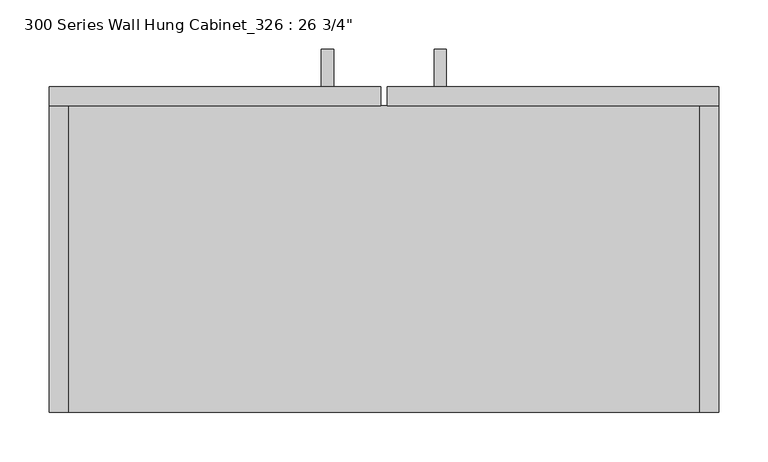
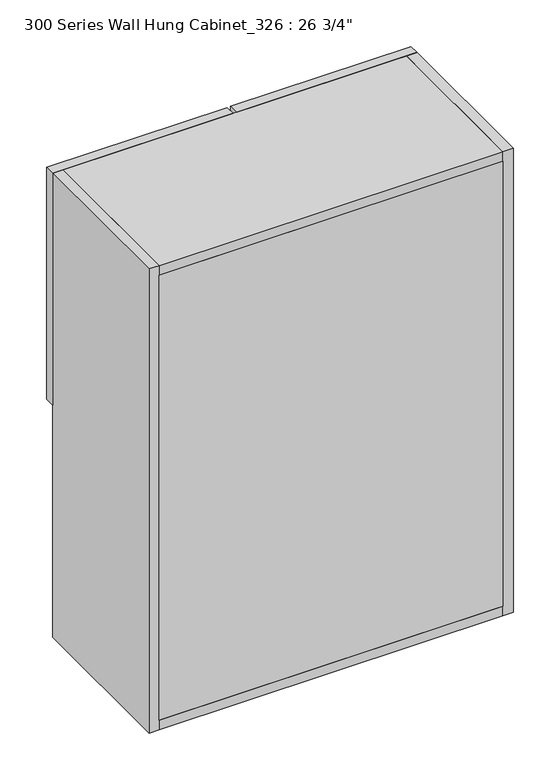
"""IFC4 building model written with IfcOpenShell, lengths in millimetres: furniture geometry."""

import ifcopenshell
import ifcopenshell.guid

model = None  # the IFC model being written
_history = None  # IfcOwnerHistory: only IFC2X3 demands one
_inside = {}  # id of a spatial element -> (the spatial element, [elements in it])
_under = {}  # id of a project, library or spatial element -> (it, [spatial elements below it])
_declared = {}  # id of a project -> (the project, [libraries it declares])
_typed = {}  # id of a type object -> (the type object, [elements of that type])
_made_of = {}  # id of a material, layer set ... -> (it, [elements and type objects made of it])


def new_model(schema):
    """Start an empty IFC model of exactly this schema.

    Asked for "IFC4X3", IfcOpenShell would pick the latest addendum, in which some entities
    have other attributes; the version numbers below select the first issue.
    IFC2X3 requires an IfcOwnerHistory on every rooted entity: one is made here for all.
    """
    global model, _history
    if schema == "IFC4X3":
        model = ifcopenshell.file(schema_version=(4, 3, 0, 0))
    else:
        model = ifcopenshell.file(schema=schema)
    _inside.clear()
    _under.clear()
    _declared.clear()
    _typed.clear()
    _made_of.clear()
    _history = None
    if model.schema == "IFC2X3":
        org = make("IfcOrganization", Name="unknown")
        user = make(
            "IfcPersonAndOrganization",
            ThePerson=make("IfcPerson", FamilyName="unknown"),
            TheOrganization=org,
        )
        app = make(
            "IfcApplication",
            ApplicationDeveloper=org,
            Version="unknown",
            ApplicationFullName="unknown",
            ApplicationIdentifier="unknown",
        )
        _history = make(
            "IfcOwnerHistory",
            OwningUser=user,
            OwningApplication=app,
            ChangeAction="ADDED",
            CreationDate=0,
        )
    return model


def make(cls, **values):
    """One entity of the class cls with the attributes given. An attribute that is None is left unset."""
    return model.create_entity(
        cls, **{name: value for name, value in values.items() if value is not None}
    )


def rooted(cls, **values):
    """An entity with a GlobalId (a new one), such as an element, a storey or a relation."""
    return make(cls, GlobalId=ifcopenshell.guid.new(), OwnerHistory=_history, **values)


def si_unit(unit_type, name, prefix=None):
    """IfcSIUnit, for example si_unit("LENGTHUNIT", "METRE", prefix="MILLI")."""
    return make("IfcSIUnit", UnitType=unit_type, Prefix=prefix, Name=name)


def assignment(units):
    """IfcUnitAssignment: the units of a project."""
    return None if units is None else make("IfcUnitAssignment", Units=units)


def point(xyz):
    """IfcCartesianPoint."""
    return None if xyz is None else make("IfcCartesianPoint", Coordinates=xyz)


def direction(xyz):
    """IfcDirection."""
    return None if xyz is None else make("IfcDirection", DirectionRatios=xyz)


def frame(location, z_axis=None, x_axis=None):
    """IfcAxis2Placement3D, a coordinate frame: its origin and axes. An axis left out is left unset."""
    return make(
        "IfcAxis2Placement3D",
        Location=point(location),
        Axis=direction(z_axis),
        RefDirection=direction(x_axis),
    )


def origin():
    """The frame at (0, 0, 0) with its axes left unset."""
    return frame((0.0, 0.0, 0.0))


def place(relative_to, where):
    """IfcLocalPlacement: puts the frame where relative to a parent placement (None: the world)."""
    return make(
        "IfcLocalPlacement", PlacementRelTo=relative_to, RelativePlacement=where
    )


def context(
    kind, dimensions, precision=None, world=None, true_north=None, identifier=None
):
    """IfcGeometricRepresentationContext, for example the 3D "Model" context."""
    return make(
        "IfcGeometricRepresentationContext",
        ContextIdentifier=identifier,
        ContextType=kind,
        CoordinateSpaceDimension=dimensions,
        Precision=precision,
        WorldCoordinateSystem=world,
        TrueNorth=true_north,
    )


def project(units=None, contexts=None):
    """IfcProject with its units and contexts."""
    return rooted(
        "IfcProject",
        Name="project",
        RepresentationContexts=contexts,
        UnitsInContext=assignment(units),
    )


def spatial(cls, under=None, at=None, **own):
    """A site, building, storey or space (cls), placed at a placement, below another one or the project."""
    s = rooted(cls, ObjectPlacement=at, **own)
    if under is not None:
        _under.setdefault(under.id(), (under, []))[1].append(s)
    return s


def polyline(points):
    """IfcPolyline through the points."""
    return make("IfcPolyline", Points=[point(p) for p in points])


def outline(outer, holes=None, kind="AREA"):
    """IfcArbitraryClosedProfileDef: a profile drawn as a closed curve; with holes, ...WithVoids."""
    if holes is None:
        return make("IfcArbitraryClosedProfileDef", ProfileType=kind, OuterCurve=outer)
    return make(
        "IfcArbitraryProfileDefWithVoids",
        ProfileType=kind,
        OuterCurve=outer,
        InnerCurves=holes,
    )


def extrude(swept, where, along, depth):
    """IfcExtrudedAreaSolid: the profile swept, set in the frame where, extruded along a direction by depth."""
    return make(
        "IfcExtrudedAreaSolid",
        SweptArea=swept,
        Position=where,
        ExtrudedDirection=direction(along),
        Depth=depth,
    )


def shape(context_of_items, identifier, shape_type, items):
    """IfcShapeRepresentation: the items that make up one representation, for example the "Body"."""
    return make(
        "IfcShapeRepresentation",
        ContextOfItems=context_of_items,
        RepresentationIdentifier=identifier,
        RepresentationType=shape_type,
        Items=items,
    )


def source(mapping_origin, context_of_items, identifier, shape_type, items):
    """IfcRepresentationMap: a shape defined once, which mapped items show again and again."""
    return make(
        "IfcRepresentationMap",
        MappingOrigin=mapping_origin,
        MappedRepresentation=shape(context_of_items, identifier, shape_type, items),
    )


def transform(
    local_origin,
    x_axis=None,
    y_axis=None,
    z_axis=None,
    scale=None,
    scale2=None,
    scale3=None,
    uniform=True,
):
    """IfcCartesianTransformationOperator3D, or its non-uniform kind. x_axis, y_axis, z_axis: its Axis1, 2, 3."""
    if uniform:
        return make(
            "IfcCartesianTransformationOperator3D",
            Axis1=direction(x_axis),
            Axis2=direction(y_axis),
            LocalOrigin=point(local_origin),
            Scale=scale,
            Axis3=direction(z_axis),
        )
    return make(
        "IfcCartesianTransformationOperator3DnonUniform",
        Axis1=direction(x_axis),
        Axis2=direction(y_axis),
        LocalOrigin=point(local_origin),
        Scale=scale,
        Axis3=direction(z_axis),
        Scale2=scale2,
        Scale3=scale3,
    )


def mapped(mapping_source, mapping_target):
    """IfcMappedItem: shows the shape of a source again, moved by a transform."""
    return make(
        "IfcMappedItem", MappingSource=mapping_source, MappingTarget=mapping_target
    )


def made_of(thing, what):
    """Note that an element or type object is made of a material, layer set ...; save() writes the relation."""
    if what is not None:
        _made_of.setdefault(what.id(), (what, []))[1].append(thing)
    return thing


def element(
    cls,
    number,
    at=None,
    inside=None,
    cuts=None,
    type_object=None,
    material=None,
    context=None,
    identifier="Body",
    shape_type=None,
    held_by="IfcProductDefinitionShape",
    body=None,
    shapes=None,
    **own,
):
    """One element of the class cls, such as IfcWall. Its Tag is "e" and its number.

    at: its placement. inside: the storey or other place that contains it. cuts: it is an
    opening in that element (IfcRelVoidsElement). A single representation is given by context,
    identifier, shape_type and body (its items); several are given by shapes. held_by: the class
    of the entity that holds the representations. save() writes the other relations.
    """
    e = rooted(cls, Tag="e%d" % number, ObjectPlacement=at, **own)
    if body is not None:
        shapes = [shape(context, identifier, shape_type, body)]
    if shapes is not None:
        e.Representation = make(held_by, Representations=shapes)
    if inside is not None:
        _inside.setdefault(inside.id(), (inside, []))[1].append(e)
    if cuts is not None:
        rooted(
            "IfcRelVoidsElement", RelatingBuildingElement=cuts, RelatedOpeningElement=e
        )
    if type_object is not None:
        _typed.setdefault(type_object.id(), (type_object, []))[1].append(e)
    return made_of(e, material)


def aggregate(whole, parts):
    """IfcRelAggregates: a whole, such as a stair, and the parts it consists of."""
    return rooted("IfcRelAggregates", RelatingObject=whole, RelatedObjects=parts)


def save(model, path):
    """Write the relations noted so far, then the file.

    IfcRelAggregates (storeys below a building ...), IfcRelContainedInSpatialStructure (elements
    in a storey), IfcRelDefinesByType, IfcRelAssociatesMaterial and IfcRelDeclares: one each for
    every whole, place, type object, material and project.
    """
    for whole, parts in _under.values():
        aggregate(whole, parts)
    for where, things in _inside.values():
        rooted(
            "IfcRelContainedInSpatialStructure",
            RelatedElements=things,
            RelatingStructure=where,
        )
    for kind, things in _typed.values():
        rooted("IfcRelDefinesByType", RelatedObjects=things, RelatingType=kind)
    for what, things in _made_of.values():
        rooted("IfcRelAssociatesMaterial", RelatedObjects=things, RelatingMaterial=what)
    for by, libraries in _declared.values():
        rooted("IfcRelDeclares", RelatingContext=by, RelatedDefinitions=libraries)
    model.write(path)


def furniture_b195cdbb(model_context):
    return source(origin(), model_context, "Body", "SweptSolid", [
        extrude(outline(polyline([(406.4, 1809.7425373), (406.4, 1822.4121874), (444.4810937, 1822.4121874), (444.4810937, 1727.2), (406.4, 1727.2), (406.4, 1739.8696501), (431.8114436, 1739.8696501), (431.8114436, 1809.7425373), (406.4, 1809.7425373)])), frame((50.8, 0.0, 0.0), z_axis=(1.0, 0.0, 0.0), x_axis=(0.0, 1.0, 0.0)), (0.0, 0.0, 1.0), 12.4065288),
        extrude(outline(polyline([(406.4, 1809.7425373), (406.4, 1822.4121874), (444.4810937, 1822.4121874), (444.4810937, 1727.2), (406.4, 1727.2), (406.4, 1739.8696501), (431.8114436, 1739.8696501), (431.8114436, 1809.7425373), (406.4, 1809.7425373)])), frame((-63.5, 0.0, 0.0), z_axis=(1.0, 0.0, 0.0), x_axis=(0.0, 1.0, 0.0)), (0.0, 0.0, 1.0), 12.4065288),
        extrude(outline(polyline([(320.675, 387.35), (320.675, 95.25), (-320.675, 95.25), (-320.675, 387.35), (320.675, 387.35)])), frame((0.0, 0.0, 1676.4), z_axis=(0.0, 0.0, 1.0), x_axis=(1.0, 0.0, 0.0)), (0.0, 0.0, 1.0), 19.05),
        extrude(outline(polyline([(320.675, 76.2), (-320.675, 76.2), (-320.675, 95.25), (320.675, 95.25), (320.675, 76.2)])), frame((0.0, 0.0, 1238.25), z_axis=(0.0, 0.0, 1.0), x_axis=(1.0, 0.0, 0.0)), (0.0, 0.0, 1.0), 876.3),
        extrude(outline(polyline([(-3.175, 387.35), (-339.725, 387.35), (-339.725, 406.4), (-3.175, 406.4), (-3.175, 387.35)])), frame((0.0, 0.0, 1676.4), z_axis=(0.0, 0.0, 1.0), x_axis=(1.0, 0.0, 0.0)), (0.0, 0.0, 1.0), 457.2),
        extrude(outline(polyline([(339.725, 387.35), (3.175, 387.35), (3.175, 406.4), (339.725, 406.4), (339.725, 387.35)])), frame((0.0, 0.0, 1676.4), z_axis=(0.0, 0.0, 1.0), x_axis=(1.0, 0.0, 0.0)), (0.0, 0.0, 1.0), 457.2),
        extrude(outline(polyline([(-339.725, 76.2), (-339.725, 387.35), (-320.675, 387.35), (-320.675, 76.2), (-339.725, 76.2)])), frame((0.0, 0.0, 1219.2), z_axis=(0.0, 0.0, 1.0), x_axis=(1.0, 0.0, 0.0)), (0.0, 0.0, 1.0), 914.4),
        extrude(outline(polyline([(320.675, 76.2), (320.675, 387.35), (339.725, 387.35), (339.725, 76.2), (320.675, 76.2)])), frame((0.0, 0.0, 1219.2), z_axis=(0.0, 0.0, 1.0), x_axis=(1.0, 0.0, 0.0)), (0.0, 0.0, 1.0), 914.4),
        extrude(outline(polyline([(320.675, 387.35), (320.675, 76.2), (-320.675, 76.2), (-320.675, 387.35), (320.675, 387.35)])), frame((0.0, 0.0, 2114.55), z_axis=(0.0, 0.0, 1.0), x_axis=(1.0, 0.0, 0.0)), (0.0, 0.0, 1.0), 19.05),
        extrude(outline(polyline([(320.675, 387.35), (320.675, 76.2), (-320.675, 76.2), (-320.675, 387.35), (320.675, 387.35)])), frame((0.0, 0.0, 1219.2), z_axis=(0.0, 0.0, 1.0), x_axis=(1.0, 0.0, 0.0)), (0.0, 0.0, 1.0), 19.05),
    ])


if __name__ == "__main__":
    model = new_model("IFC4")
    model_context = context("Model", 3, world=origin())
    ifc_project = project(units=[si_unit("LENGTHUNIT", "METRE", prefix="MILLI")], contexts=[model_context])
    site = spatial("IfcSite", under=ifc_project)
    building = spatial("IfcBuilding", under=site)
    placement = place(None, origin())
    furniture_shape = furniture_b195cdbb(model_context)
    element("IfcFurniture", 1, ObjectType="300 Series Wall Hung Cabinet_326 : 26 3/4\"", at=placement, inside=building, context=model_context, shape_type="MappedRepresentation", body=[
        mapped(furniture_shape, transform((0.0, 0.0, 0.0), x_axis=(1.0, 0.0, 0.0), y_axis=(0.0, 1.0, 0.0), z_axis=(0.0, 0.0, 1.0))),
    ])
    save(model, "model.ifc")

# Revit data of these elements
# Type "300 Series Wall Hung Cabinet_326 : 26 3/4\""
#   URL = "www.wicnet.org/manual_sections.asp"
#   Model = "326"
#   Manufacturer = "Woodwork Institute"
#   Content Creator URL = "www.AECcontent.com"
#   Content Creator = "AECcontent"
#   Description = "Wall Hung Cabinet"
#   Assembly Code = "E2010200"
#   Width = 2' - 2 3/4"
#   Top of Cabinet = 7' - 0"
#   Height = 3' - 0"
#   Depth = 1' - 1"
#   Top Panel Material = Cabinet
#   Side Panel Material = Cabinet
#   Shelf Panel Material = Cabinet
#   Back Panel Material = Cabinet
#   Door Panel Material = Cabinet
# Element 1 (IfcFurniture, "300 Series Wall Hung Cabinet_326 : 26 3/4\"")
#   Materials on its faces: "Cabinet", "Default metal"
# Materials
#   "Cabinet": class "Wood", colour RGB 189 170 130, transparency 0, Cost = 0
#   "Default metal": class "Unassigned", colour RGB 204 204 204, transparency 0
